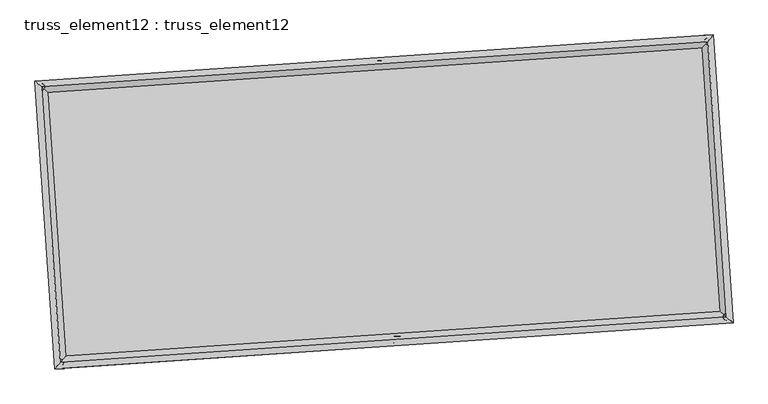
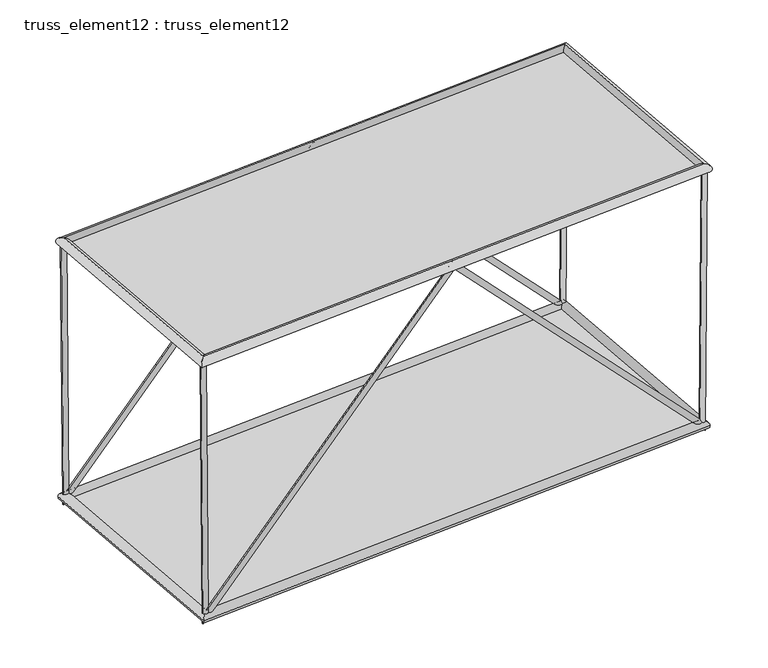
"""IFC4 building model written with IfcOpenShell, lengths in millimetres: plate geometry, truss_element12 : truss_element12."""

from ifc_helpers import new_model, si_unit, frame, origin, origin_with_axes, place, context, project, spatial, polyline, circle_curve, ellipse_curve, outline, extrude, source, transform, mapped, element, save
from ifc_brep_helpers import plane_surface, cylinder_surface, advanced_brep


def truss_element12_truss_element12_cb063575(model_context):
    return source(origin(), model_context, "Body", "SolidModel", [
        advanced_brep(
        [(-3704.5695702, 2273.5219079, 5000.2385631), (-3803.6697911, 2260.160847, 4999.445924), (-3665.9165394, 2276.1575111, 123.1909224), (-3763.0703435, 2262.929169, -123.1909224), (1063.3965363, 2598.6313919, 5071.9675621), (1063.8495614, 2592.0584884, 4927.7219872), (5793.3396752, 2921.1482344, 123.1954626), (5891.4213018, 2921.2322541, -123.1954626), (5831.3674137, 2923.7412013, 5000.2372149), (5931.3641428, 2923.9558046, 4999.4573967)],
        [
            (0, 1, circle_curve(frame((-3754.1196806, 2266.8413774, 4999.8422436), z_axis=(-0.00792524784066047, -0.0005403925235671604, 0.9999684487135504), x_axis=(-0.13361067680332622, 0.9910337598342116, -0.0005233670063100185)), 50.0)),
            (1, 0, circle_curve(frame((-3754.1196806, 2266.8413774, 4999.8422436), z_axis=(-0.00792524784066047, -0.0005403925235671604, 0.9999684487135504), x_axis=(-0.13361067680332622, 0.9910337598342116, -0.0005233670063100185)), 50.0)),
            (0, 2),
            (2, 3, ellipse_curve(frame((-3714.4934414, 2269.54334, 0.0), z_axis=(-0.9272625104149091, -0.06322650573039987, 0.369034748705544), x_axis=(0.3681798413581857, 0.02510478379961125, 0.9294155982378585)), 132.8352693, 50.0)),
            (3, 1),
            (3, 2, ellipse_curve(frame((-3714.4934414, 2269.54334, 0.0), z_axis=(-0.9272625104149091, -0.06322650573039987, 0.369034748705544), x_axis=(0.3681798413581857, 0.02510478379961125, 0.9294155982378585)), 132.8352693, 50.0)),
            (2, 4),
            (4, 5, ellipse_curve(frame((1063.6230488, 2595.3449402, 4999.8447747), z_axis=(-0.997683395514968, -0.06802823819052738, -3.35024863646144e-05), x_axis=(3.342487437292575e-05, 2.2791151234968384e-06, -0.9999999994387916)), 72.2798352, 50.0)),
            (5, 3),
            (5, 4, ellipse_curve(frame((1063.6230488, 2595.3449402, 4999.8447747), z_axis=(-0.997683395514968, -0.06802823819052738, -3.35024863646144e-05), x_axis=(3.342487437292575e-05, 2.2791151234968384e-06, -0.9999999994387916)), 72.2798352, 50.0)),
            (4, 6),
            (6, 7, ellipse_curve(frame((5842.3804885, 2921.1902443, 0.0), z_axis=(-0.9272265170481916, -0.06322405147954682, -0.3691255956950034), x_axis=(-0.36827047789115297, -0.025110963960252405, 0.9293795212951536)), 132.8453216, 50.0)),
            (7, 5),
            (7, 6, ellipse_curve(frame((5842.3804885, 2921.1902443, 0.0), z_axis=(-0.9272265170481916, -0.06322405147954682, -0.3691255956950034), x_axis=(-0.36827047789115297, -0.025110963960252405, 0.9293795212951536)), 132.8453216, 50.0)),
            (8, 9, circle_curve(frame((5881.3657782, 2923.848503, 4999.8473058), z_axis=(0.0077970579476175144, 0.0005316517420560585, 0.9999694611505828), x_axis=(-0.0021501131416041324, 0.9999975559419182, -0.0005149016104120452)), 50.0)),
            (9, 8, circle_curve(frame((5881.3657782, 2923.848503, 4999.8473058), z_axis=(0.0077970579476175144, 0.0005316517420560585, 0.9999694611505828), x_axis=(-0.0021501131416041324, 0.9999975559419182, -0.0005149016104120452)), 50.0)),
            (6, 8),
            (9, 7),
        ],
        [
            plane_surface(frame((-3754.1196806, 2316.8413701, 4999.869264), z_axis=(-0.00792524784066071, -0.0005403925235714989, 0.9999684487135506), x_axis=(0.9999685947301866, -4.282879185524282e-06, 0.007925246683406334))),
            cylinder_surface(frame((-3754.1196806, 2266.8413774, 4999.8422436), z_axis=(-0.007925247840660472, -0.0005403925235671605, 0.9999684487135506), x_axis=(-0.13361067680332622, 0.9910337598342116, -0.0005233670063100185)), 50.0),
            cylinder_surface(frame((-3714.4934414, 2269.54334, 0.0), z_axis=(-0.6901292038292404, -0.04705728698241158, -0.7221546190144281), x_axis=(-0.020411527938873002, 0.9987523794850289, -0.045574707900252545)), 50.0),
            cylinder_surface(frame((1063.6230488, 2595.3449402, 4999.8447747), z_axis=(-0.6901774781348256, -0.047060578623801405, 0.7221082679315101), x_axis=(-0.11534628179156464, 0.9922791395005983, -0.04557789583573464)), 50.0),
            plane_surface(frame((5881.3657782, 2873.84851, 4999.8738891), z_axis=(0.007797057947618262, 0.0005316517420571678, 0.9999694611505827), x_axis=(0.9999696024816762, -4.14544545179751e-06, -0.0077970568456180375))),
            cylinder_surface(frame((5842.3804885, 2921.1902443, 0.0), z_axis=(-0.007797057947617513, -0.0005316517420560584, -0.9999694611505826), x_axis=(-0.0021501131416041324, 0.9999975559419182, -0.0005149016104120452)), 50.0),
        ],
        [
            (0, [[1, 2]]),
            (1, [[-1, 3, 4, 5]]),
            (1, [[-2, -5, 6, -3]]),
            (2, [[-4, 7, 8, 9]]),
            (2, [[-6, -9, 10, -7]]),
            (3, [[-8, 11, 12, 13]]),
            (3, [[-10, -13, 14, -11]]),
            (4, [[15, 16]]),
            (5, [[-12, 17, -16, 18]]),
            (5, [[-14, -18, -15, -17]]),
        ],
    ),
        advanced_brep(
        [(-3432.4566173, -1717.2116764, 5000.2385631), (-3531.5568381, -1730.5727373, 4999.445924), (-3393.8035864, -1714.5760732, 123.1909224), (-3490.9573906, -1727.8044153, -123.1909224), (1335.5094892, -1392.1021924, 5071.9675621), (1335.9625143, -1398.6750959, 4927.7219872), (6065.4526281, -1069.5853499, 123.1954626), (6163.5342547, -1069.5013302, -123.1954626), (6103.4803666, -1066.992383, 5000.2372149), (6203.4770957, -1066.7777797, 4999.4573967)],
        [
            (0, 1, circle_curve(frame((-3482.0067277, -1723.8922069, 4999.8422436), z_axis=(-0.007925247840660425, -0.0005403925235671344, 0.9999684487135505), x_axis=(-0.13361067680332553, 0.9910337598342117, -0.0005233670063100326)), 50.0)),
            (1, 0, circle_curve(frame((-3482.0067277, -1723.8922069, 4999.8422436), z_axis=(-0.007925247840660425, -0.0005403925235671344, 0.9999684487135505), x_axis=(-0.13361067680332553, 0.9910337598342117, -0.0005233670063100326)), 50.0)),
            (0, 2),
            (2, 3, ellipse_curve(frame((-3442.3804885, -1721.1902443, 0.0), z_axis=(-0.9272625104149091, -0.06322650573039948, 0.36903474870554426), x_axis=(0.3681798413581859, 0.025104783799611126, 0.929415598237858)), 132.8352693, 50.0)),
            (3, 1),
            (3, 2, ellipse_curve(frame((-3442.3804885, -1721.1902443, 0.0), z_axis=(-0.9272625104149091, -0.06322650573039948, 0.36903474870554426), x_axis=(0.3681798413581859, 0.025104783799611126, 0.929415598237858)), 132.8352693, 50.0)),
            (2, 4),
            (4, 5, ellipse_curve(frame((1335.7360017, -1395.3886441, 4999.8447747), z_axis=(-0.9976833955149681, -0.06802823819052717, -3.3502486364694645e-05), x_axis=(3.342487437338699e-05, 2.2791151236986262e-06, -0.9999999994387916)), 72.2798352, 50.0)),
            (5, 3),
            (5, 4, ellipse_curve(frame((1335.7360017, -1395.3886441, 4999.8447747), z_axis=(-0.9976833955149681, -0.06802823819052717, -3.3502486364694645e-05), x_axis=(3.342487437338699e-05, 2.2791151236986262e-06, -0.9999999994387916)), 72.2798352, 50.0)),
            (4, 6),
            (6, 7, ellipse_curve(frame((6114.4934414, -1069.54334, 0.0), z_axis=(-0.9272265170481916, -0.06322405147954674, -0.36912559569500364), x_axis=(-0.3682704778911531, -0.025110963960252405, 0.9293795212951536)), 132.8453216, 50.0)),
            (7, 5),
            (7, 6, ellipse_curve(frame((6114.4934414, -1069.54334, 0.0), z_axis=(-0.9272265170481916, -0.06322405147954674, -0.36912559569500364), x_axis=(-0.3682704778911531, -0.025110963960252405, 0.9293795212951536)), 132.8453216, 50.0)),
            (8, 9, circle_curve(frame((6153.4787312, -1066.8850813, 4999.8473058), z_axis=(0.007797057947617367, 0.0005316517420560059, 0.9999694611505828), x_axis=(-0.0021501131416044885, 0.9999975559419183, -0.0005149016104119903)), 50.0)),
            (9, 8, circle_curve(frame((6153.4787312, -1066.8850813, 4999.8473058), z_axis=(0.007797057947617367, 0.0005316517420560059, 0.9999694611505828), x_axis=(-0.0021501131416044885, 0.9999975559419183, -0.0005149016104119903)), 50.0)),
            (6, 8),
            (9, 7),
        ],
        [
            plane_surface(frame((-3482.0067277, -1673.8922142, 4999.869264), z_axis=(-0.00792524784066071, -0.0005403925235715033, 0.9999684487135506), x_axis=(0.9999685947301866, -4.282879185524282e-06, 0.007925246683406334))),
            cylinder_surface(frame((-3482.0067277, -1723.8922069, 4999.8422436), z_axis=(-0.007925247840660425, -0.0005403925235671344, 0.9999684487135505), x_axis=(-0.13361067680332553, 0.9910337598342117, -0.0005233670063100326)), 50.0),
            cylinder_surface(frame((-3442.3804885, -1721.1902443, 0.0), z_axis=(-0.6901292038292406, -0.04705728698241133, -0.7221546190144281), x_axis=(-0.02041152793887286, 0.998752379485029, -0.04557470790025232)), 50.0),
            cylinder_surface(frame((1335.7360017, -1395.3886441, 4999.8447747), z_axis=(-0.6901774781348259, -0.04706057862380139, 0.7221082679315098), x_axis=(-0.11534628179156436, 0.9922791395005984, -0.04557789583573443)), 50.0),
            plane_surface(frame((6153.4787312, -1116.8850743, 4999.8738891), z_axis=(0.007797057947618262, 0.0005316517420571736, 0.9999694611505827), x_axis=(0.9999696024816762, -4.14544545179751e-06, -0.0077970568456180375))),
            cylinder_surface(frame((6114.4934414, -1069.54334, 0.0), z_axis=(-0.007797057947617367, -0.0005316517420560059, -0.9999694611505828), x_axis=(-0.0021501131416044885, 0.9999975559419183, -0.0005149016104119903)), 50.0),
        ],
        [
            (0, [[1, 2]]),
            (1, [[-1, 3, 4, 5]]),
            (1, [[-2, -5, 6, -3]]),
            (2, [[-4, 7, 8, 9]]),
            (2, [[-6, -9, 10, -7]]),
            (3, [[-8, 11, 12, 13]]),
            (3, [[-10, -13, 14, -11]]),
            (4, [[15, 16]]),
            (5, [[-12, 17, -16, 18]]),
            (5, [[-14, -18, -15, -17]]),
        ],
    ),
        advanced_brep(
        [(-3482.0053928, -1723.8907274, 4909.8422436), (-3482.0080626, -1723.8936864, 5089.8422436), (-3754.121204, 2266.8426621, 5089.8422436), (-3754.1181572, 2266.8400928, 4909.8422436), (5881.367019, 2923.8499761, 5089.8473057), (5881.3645375, 2923.8470299, 4909.8473058), (6153.4801604, -1066.8863724, 5089.8473057), (6153.4773019, -1066.8837903, 4909.8473058)],
        [
            (0, 1, ellipse_curve(frame((-3482.0067277, -1723.8922069, 4999.8422436), z_axis=(-0.7535719234053619, 0.6573654662780863, -3.7063136814546204e-07), x_axis=(-0.6573654662779828, -0.7535719234054522, -3.7063136814550154e-07)), 127.2792206, 90.0)),
            (1, 2),
            (2, 3, ellipse_curve(frame((-3754.1196806, 2266.8413774, 4999.8422436), z_axis=(-0.6573654662779828, -0.7535719234054524, -3.706313681455368e-07), x_axis=(0.7535719234053622, -0.657365466278086, 3.706313681454975e-07)), 127.2792206, 90.0)),
            (3, 0),
            (1, 0, ellipse_curve(frame((-3482.0067277, -1723.8922069, 4999.8422436), z_axis=(-0.7535719234053619, 0.6573654662780863, -3.7063136814546204e-07), x_axis=(-0.6573654662779828, -0.7535719234054522, -3.7063136814550154e-07)), 127.2792206, 90.0)),
            (3, 2, ellipse_curve(frame((-3754.1196806, 2266.8413774, 4999.8422436), z_axis=(-0.6573654662779828, -0.7535719234054524, -3.706313681455368e-07), x_axis=(0.7535719234053622, -0.657365466278086, 3.706313681454975e-07)), 127.2792206, 90.0)),
            (2, 4),
            (4, 5, ellipse_curve(frame((5881.3657782, 2923.848503, 4999.8473058), z_axis=(-0.7535719234053619, 0.6573654662780863, -3.706313681455331e-07), x_axis=(-0.6573654662779828, -0.7535719234054523, -3.70631368145501e-07)), 127.2792206, 90.0)),
            (5, 3),
            (5, 4, ellipse_curve(frame((5881.3657782, 2923.848503, 4999.8473058), z_axis=(-0.7535719234053619, 0.6573654662780863, -3.706313681455331e-07), x_axis=(-0.6573654662779828, -0.7535719234054523, -3.70631368145501e-07)), 127.2792206, 90.0)),
            (4, 6),
            (6, 7, ellipse_curve(frame((6153.4787312, -1066.8850813, 4999.8473058), z_axis=(0.6573654662779831, 0.7535719234054521, 3.7063136814546586e-07), x_axis=(-0.7535719234053616, 0.6573654662780866, -3.706313681454977e-07)), 127.2792206, 90.0)),
            (7, 5),
            (7, 6, ellipse_curve(frame((6153.4787312, -1066.8850813, 4999.8473058), z_axis=(0.6573654662779831, 0.7535719234054521, 3.7063136814546586e-07), x_axis=(-0.7535719234053616, 0.6573654662780866, -3.706313681454977e-07)), 127.2792206, 90.0)),
            (6, 1),
            (0, 7),
        ],
        [
            cylinder_surface(frame((-3482.0067277, -1723.8922069, 4999.8422436), z_axis=(0.06802823822870381, -0.9976833960748765, 0.0), x_axis=(-0.9976833959485082, -0.06802823822008723, -1.5916136027239472e-05)), 90.0),
            cylinder_surface(frame((-3754.1196806, 2266.8413774, 4999.8422436), z_axis=(-0.9976833960747395, -0.0680282382286924, -5.241519074722858e-07), x_axis=(-0.06802823821259431, 0.9976833959572432, -1.5391984119829294e-05)), 90.0),
            cylinder_surface(frame((5881.3657782, 2923.848503, 4999.8473058), z_axis=(-0.06802823822870332, 0.9976833960748764, 0.0), x_axis=(0.9976833959646063, 0.06802823822118442, -1.4867832212419123e-05)), 90.0),
            cylinder_surface(frame((6153.4787312, -1066.8850813, 4999.8473058), z_axis=(0.9976833960747397, 0.06802823822869221, 5.241519074722359e-07), x_axis=(0.06802823822869221, -0.9976833959561456, -1.53919841198293e-05)), 90.0),
        ],
        [
            (0, [[1, 2, 3, 4]]),
            (0, [[5, -4, 6, -2]]),
            (1, [[-3, 7, 8, 9]]),
            (1, [[-6, -9, 10, -7]]),
            (2, [[-8, 11, 12, 13]]),
            (2, [[-10, -13, 14, -11]]),
            (3, [[-12, 15, -1, 16]]),
            (3, [[-14, -16, -5, -15]]),
        ],
    ),
        advanced_brep(
        [(-3358.7115243, -1625.2761972, 0.0), (-3526.0494527, -1817.1042913, 0.0), (-3810.4074885, 2353.2123043, 0.0), (-3618.5793943, 2185.8743758, 0.0), (5926.0494527, 3017.1042913, 0.0), (5758.7115243, 2825.2761972, 0.0), (6210.4074885, -1153.2123043, 0.0), (6018.5793943, -985.8743758, 0.0)],
        [
            (0, 1, ellipse_curve(frame((-3442.3804885, -1721.1902443, 0.0), z_axis=(-0.7535719234054611, 0.6573654662780772, 0.0), x_axis=(-0.6573654662780772, -0.753571923405461, 0.0)), 127.2792206, 90.0)),
            (1, 2),
            (2, 3, ellipse_curve(frame((-3714.4934414, 2269.54334, 0.0), z_axis=(-0.6573654662780771, -0.7535719234054612, 0.0), x_axis=(0.7535719234054612, -0.6573654662780772, 0.0)), 127.2792206, 90.0)),
            (3, 0),
            (1, 0, ellipse_curve(frame((-3442.3804885, -1721.1902443, 0.0), z_axis=(-0.7535719234054611, 0.6573654662780772, 0.0), x_axis=(-0.6573654662780772, -0.753571923405461, 0.0)), 127.2792206, 90.0)),
            (3, 2, ellipse_curve(frame((-3714.4934414, 2269.54334, 0.0), z_axis=(-0.6573654662780771, -0.7535719234054612, 0.0), x_axis=(0.7535719234054612, -0.6573654662780772, 0.0)), 127.2792206, 90.0)),
            (2, 4),
            (4, 5, ellipse_curve(frame((5842.3804885, 2921.1902443, 0.0), z_axis=(-0.7535719234054612, 0.6573654662780772, 0.0), x_axis=(-0.657365466278077, -0.7535719234054612, 0.0)), 127.2792206, 90.0)),
            (5, 3),
            (5, 4, ellipse_curve(frame((5842.3804885, 2921.1902443, 0.0), z_axis=(-0.7535719234054612, 0.6573654662780772, 0.0), x_axis=(-0.657365466278077, -0.7535719234054612, 0.0)), 127.2792206, 90.0)),
            (4, 6),
            (6, 7, ellipse_curve(frame((6114.4934414, -1069.54334, 0.0), z_axis=(0.6573654662780773, 0.753571923405461, 0.0), x_axis=(-0.7535719234054611, 0.6573654662780773, 0.0)), 127.2792206, 90.0)),
            (7, 5),
            (7, 6, ellipse_curve(frame((6114.4934414, -1069.54334, 0.0), z_axis=(0.6573654662780773, 0.753571923405461, 0.0), x_axis=(-0.7535719234054611, 0.6573654662780773, 0.0)), 127.2792206, 90.0)),
            (6, 1),
            (0, 7),
        ],
        [
            cylinder_surface(frame((-3442.3804885, -1721.1902443, 0.0), z_axis=(0.06802823822870709, -0.9976833960748762, 0.0), x_axis=(-0.9976833960748762, -0.06802823822870709, 0.0)), 90.0),
            cylinder_surface(frame((-3714.4934414, 2269.54334, 0.0), z_axis=(-0.9976833960748763, -0.06802823822870516, 0.0), x_axis=(-0.06802823822870516, 0.9976833960748763, 0.0)), 90.0),
            cylinder_surface(frame((5842.3804885, 2921.1902443, 0.0), z_axis=(-0.06802823822870689, 0.9976833960748762, 0.0), x_axis=(0.9976833960748762, 0.06802823822870689, 0.0)), 90.0),
            cylinder_surface(frame((6114.4934414, -1069.54334, 0.0), z_axis=(0.9976833960748763, 0.06802823822870482, 0.0), x_axis=(0.06802823822870482, -0.9976833960748763, 0.0)), 90.0),
        ],
        [
            (0, [[1, 2, 3, 4]]),
            (0, [[5, -4, 6, -2]]),
            (1, [[-3, 7, 8, 9]]),
            (1, [[-6, -9, 10, -7]]),
            (2, [[-8, 11, 12, 13]]),
            (2, [[-10, -13, 14, -11]]),
            (3, [[-12, 15, -1, 16]]),
            (3, [[-14, -16, -5, -15]]),
        ],
    ),
        extrude(outline(polyline([(-3442.3804885, -1721.1902443), (-3714.4934414, 2269.54334), (5842.3804885, 2921.1902443), (6114.4934414, -1069.54334), (-3442.3804885, -1721.1902443)])), origin_with_axes(), (0.0, 0.0, 1.0), 20.0),
        extrude(outline(polyline([(-2000.0, 4828.9294464), (2000.0, 4828.9294464), (2000.0000001, -4828.9294463), (-1999.9999999, -4828.9294464), (-2000.0, 4828.9294464)])), frame((1199.6795253, 599.978148, 4999.8447747), z_axis=(-5.229376551060489e-07, -3.5657130829554225e-08, 0.9999999999998627), x_axis=(-0.06802823822870722, 0.9976833960748762, 0.0)), (0.0, 0.0, 1.0), 20.0),
    ])


if __name__ == "__main__":
    model = new_model("IFC4")
    model_context = context("Model", 3, world=origin())
    ifc_project = project(units=[si_unit("LENGTHUNIT", "METRE", prefix="MILLI")], contexts=[model_context])
    site = spatial("IfcSite", under=ifc_project)
    building = spatial("IfcBuilding", under=site)
    placement = place(None, origin())
    truss_element12_truss_element12_shape = truss_element12_truss_element12_cb063575(model_context)
    element("IfcPlate", 1, ObjectType="truss_element12 : truss_element12", at=placement, inside=building, context=model_context, shape_type="MappedRepresentation", body=[
        mapped(truss_element12_truss_element12_shape, transform((0.0, 0.0, 0.0), x_axis=(1.0, 0.0, 0.0), y_axis=(0.0, 1.0, 0.0), z_axis=(0.0, 0.0, 1.0))),
    ])
    save(model, "model.ifc")

# Revit data of these elements
# Type "truss_element12 : truss_element12"
#   steellbar1 = 90 mm
#   steelbar2 = 50 mm
#   offset1 = 5000 mm
#   M = Default Roof
# Element 1 (IfcPlate, "truss_element12 : truss_element12")
#   Materials on its faces: "Default Roof"
# Materials
#   "Default Roof": class "Miscellaneous", colour RGB 0 127 0, transparency 0, Comments = "Rendering appearance not upgraded Rendering appearance not upgraded ", Cost = 0
